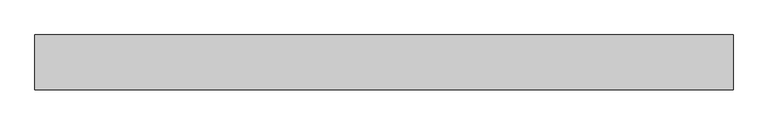
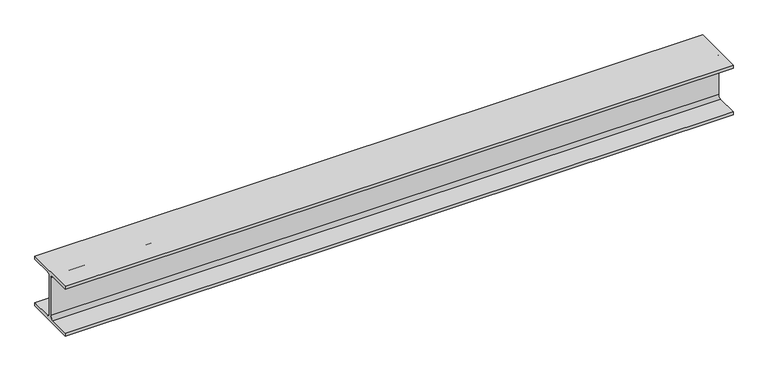
"""IFC4 building model written with IfcOpenShell, lengths in millimetres: beam geometry, 0912_Steel Framing_H-KSD3502 : H_SB_ASB_H-200x200x8x12."""

from ifc_helpers import new_model, si_unit, point, frame, frame_2d, origin, place, context, project, spatial, polyline, circle_curve, trimmed, segment, composite_curve, outline, extrude, source, transform, mapped, element, save


def beam_e6e7ec7e(model_context):
    return source(origin(), model_context, "Body", "SweptSolid", [
        extrude(outline(composite_curve([segment(polyline([(100.0, -88.0), (100.0, -100.0), (-100.0, -100.0), (-100.0, -88.0), (-17.0, -88.0)]), True, "CONTINUOUS"), segment(trimmed(circle_curve(frame_2d((-17.0, -75.0)), 13.0), [point((-17.0, -88.0))], [point((-4.0, -75.0))], True, "CARTESIAN"), True, "CONTINUOUS"), segment(polyline([(-4.0, -75.0), (-4.0, 75.0)]), True, "CONTINUOUS"), segment(trimmed(circle_curve(frame_2d((-17.0, 75.0)), 13.0), [point((-4.0, 75.0))], [point((-17.0, 88.0))], True, "CARTESIAN"), True, "CONTINUOUS"), segment(polyline([(-17.0, 88.0), (-100.0, 88.0), (-100.0, 100.0), (100.0, 100.0), (100.0, 88.0), (17.0, 88.0)]), True, "CONTINUOUS"), segment(trimmed(circle_curve(frame_2d((17.0, 75.0)), 13.0), [point((17.0, 88.0))], [point((4.0, 75.0))], True, "CARTESIAN"), True, "CONTINUOUS"), segment(polyline([(4.0, 75.0), (4.0, -75.0)]), True, "CONTINUOUS"), segment(trimmed(circle_curve(frame_2d((17.0, -75.0)), 13.0), [point((4.0, -75.0))], [point((17.0, -88.0))], True, "CARTESIAN"), True, "CONTINUOUS"), segment(polyline([(17.0, -88.0), (100.0, -88.0)]), True, "CONTINUOUS")], self_intersect=False)), frame((-1259.7617812, 0.0, 0.0), z_axis=(1.0, 0.0, 0.0), x_axis=(0.0, 1.0, 0.0)), (0.0, 0.0, 1.0), 2537.8147919),
    ])


if __name__ == "__main__":
    model = new_model("IFC4")
    model_context = context("Model", 3, world=origin())
    ifc_project = project(units=[si_unit("LENGTHUNIT", "METRE", prefix="MILLI")], contexts=[model_context])
    site = spatial("IfcSite", under=ifc_project)
    building = spatial("IfcBuilding", under=site)
    placement = place(None, origin())
    beam_shape = beam_e6e7ec7e(model_context)
    element("IfcBeam", 1, ObjectType="0912_Steel Framing_H-KSD3502 : H_SB_ASB_H-200x200x8x12", at=placement, inside=building, context=model_context, shape_type="MappedRepresentation", body=[
        mapped(beam_shape, transform((0.0, 0.0, 0.0), x_axis=(1.0, 0.0, 0.0), y_axis=(0.0, 1.0, 0.0), z_axis=(0.0, 0.0, 1.0))),
    ])
    save(model, "model.ifc")

# Revit data of these elements
# Type "0912_Steel Framing_H-KSD3502 : H_SB_ASB_H-200x200x8x12"
#   H_WM Code_1 = "S01AA002-00001 | Main Steel Structure Fabrication Work | Shelter/Building | Medium Steel - Standard (90KG/M>Weight≥30KG/M) | Material: (   )"
#   H_WM Code_2 = "S03AA028-00001 | Main Steel Structure Erection Work | Shelter/Building | Medium Steel (90KG/M>Weight≥30KG/M) | Material: (   )"
#   H_WM Code_3 = "S01AA010-00001 | Main Steel Structure Fabrication Work | Shelter/Building | Steel Painting/Coating | for Non-Fireproofed Steel Surface, Surface Preparation, Primer, Second & Final Coat | Material: (   )"
#   H_Q'ty Cal Type Tag = "SB-Q2"
#   Width = 20.0 cm
#   Web Thickness = 0.8 cm
#   Web Fillet = 1.3 cm
#   Warping Constant = 141000.0 cm⁶
#   W = 0
#   Torsional Moment of Inertia = 26.2485 cm⁴
#   Section Area = 63.53 cm²
#   Plastic Modulus weak axis = 244.0 cm³
#   Plastic Modulus strong axis = 525.0 cm³
#   Perimeter = 1.16 m²/m
#   Nominal Weight = 49.90 kgf/m
#   Moment of Inertia weak axis = 1600.00 cm⁴
#   Moment of Inertia strong axis = 4720.00 cm⁴
#   Height = 20.0 cm
#   Flange Thickness = 1.2 cm
#   Elastic Modulus weak axis = 160.0 cm³
#   Elastic Modulus strong axis = 472.0 cm³
#   Centroid Vertical = 10.0 cm
#   Centroid Horizontal = 10.0 cm
#   Ix = 47200000
#   Length [instance default] = 1.5240 m
#   Zx = 525000
#   b = 0.2000 m
#   h = 0.2000 m
#   r = 0.0130 m
#   s = 0.0080 m
#   t = 0.0120 m
#   A = 0.006353 m²
#   Structural Material [instance default] = Steel, 45-345
#   Assembly Code = ""
# Element 1 (IfcBeam, "0912_Steel Framing_H-KSD3502 : H_SB_ASB_H-200x200x8x12")
#   Structural Material = none
# Materials
#   "Steel, 45-345": class "Metal", colour RGB 189 187 185, transparency 0, Description = "Steel 345 MPa", Cost = 0
